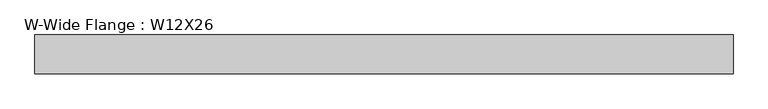
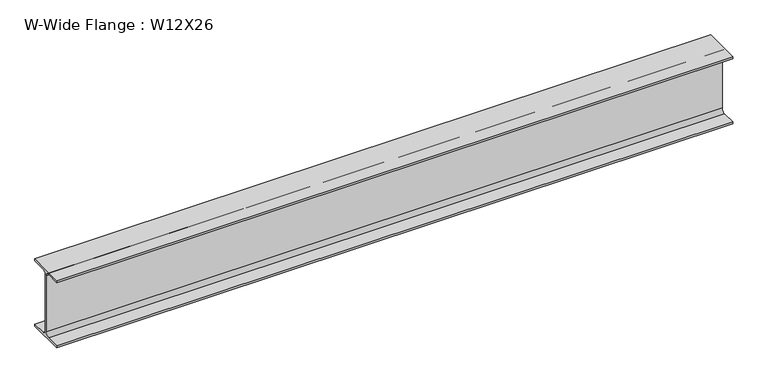
"""IFC4 building model written with IfcOpenShell, lengths in millimetres: beam geometry, W-Wide Flange : W12X26."""

from ifc_helpers import new_model, si_unit, point, frame, frame_2d, origin, place, context, project, spatial, polyline, circle_curve, trimmed, segment, composite_curve, outline, extrude, source, transform, mapped, element, save


def w_wide_flange_w12x26_35e54b53(model_context):
    return source(origin(), model_context, "Body", "SweptSolid", [
        extrude(outline(composite_curve([segment(polyline([(82.423, -145.288), (82.423, -154.94), (-82.423, -154.94), (-82.423, -145.288), (-20.2565, -145.288)]), True, "CONTINUOUS"), segment(trimmed(circle_curve(frame_2d((-20.2565, -127.9525)), 17.3355), [point((-20.2565, -145.288))], [point((-2.921, -127.9525))], True, "CARTESIAN"), True, "CONTINUOUS"), segment(polyline([(-2.921, -127.9525), (-2.921, 127.9525)]), True, "CONTINUOUS"), segment(trimmed(circle_curve(frame_2d((-20.2565, 127.9525)), 17.3355), [point((-2.921, 127.9525))], [point((-20.2565, 145.288))], True, "CARTESIAN"), True, "CONTINUOUS"), segment(polyline([(-20.2565, 145.288), (-82.423, 145.288), (-82.423, 154.94), (82.423, 154.94), (82.423, 145.288), (20.2565, 145.288)]), True, "CONTINUOUS"), segment(trimmed(circle_curve(frame_2d((20.2565, 127.9525)), 17.3355), [point((20.2565, 145.288))], [point((2.921, 127.9525))], True, "CARTESIAN"), True, "CONTINUOUS"), segment(polyline([(2.921, 127.9525), (2.921, -127.9525)]), True, "CONTINUOUS"), segment(trimmed(circle_curve(frame_2d((20.2565, -127.9525)), 17.3355), [point((2.921, -127.9525))], [point((20.2565, -145.288))], True, "CARTESIAN"), True, "CONTINUOUS"), segment(polyline([(20.2565, -145.288), (82.423, -145.288)]), True, "CONTINUOUS")], self_intersect=False)), frame((-1473.2, 0.0, 0.0), z_axis=(1.0, 0.0, 0.0), x_axis=(0.0, 1.0, 0.0)), (0.0, 0.0, 1.0), 2946.4),
    ])


if __name__ == "__main__":
    model = new_model("IFC4")
    model_context = context("Model", 3, world=origin())
    ifc_project = project(units=[si_unit("LENGTHUNIT", "METRE", prefix="MILLI")], contexts=[model_context])
    site = spatial("IfcSite", under=ifc_project)
    building = spatial("IfcBuilding", under=site)
    placement = place(None, origin())
    w_wide_flange_w12x26_shape = w_wide_flange_w12x26_35e54b53(model_context)
    element("IfcBeam", 1, ObjectType="W-Wide Flange : W12X26", at=placement, inside=building, context=model_context, shape_type="MappedRepresentation", body=[
        mapped(w_wide_flange_w12x26_shape, transform((0.0, 0.0, 0.0), x_axis=(1.0, 0.0, 0.0), y_axis=(0.0, 1.0, 0.0), z_axis=(0.0, 0.0, 1.0))),
    ])
    save(model, "model.ifc")

# Revit data of these elements
# Type "W-Wide Flange : W12X26"
#   Assembly Code = "B10"
#   W = 26
#   Length [instance default] = 5' - 0"
#   bf = 0' - 6.49"
#   d = 1' - 0.2"
#   k = 0' - 1 1/16"
#   k2 = 0' - 0.6825"
#   tf = 0' - 0.38"
#   tw = 0' - 0.23"
#   A = 0.053125 SF
#   Structural Material [instance default] = Steel ASTM A992
# Element 1 (IfcBeam, "W-Wide Flange : W12X26")
#   Materials on its faces: "Steel ASTM A992"
# Materials
#   "Steel ASTM A992": class "Metal", colour RGB 199 199 199, transparency 0, Description = "Structural steel 50ksi", Cost = 0
